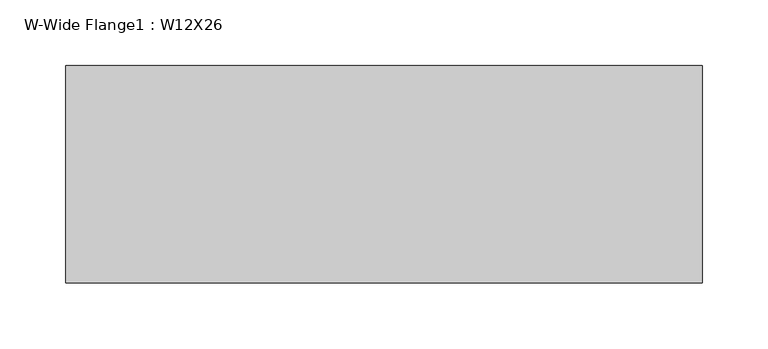
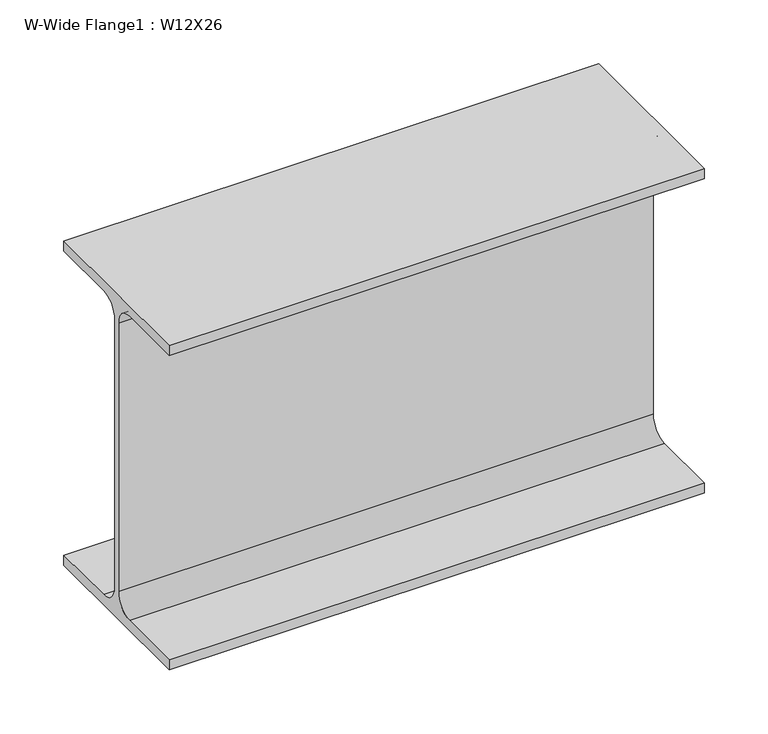
"""IFC4 building model written with IfcOpenShell, lengths in millimetres: beam geometry, W-Wide Flange1 : W12X26."""

import ifcopenshell
import ifcopenshell.guid

model = None  # the IFC model being written
_history = None  # IfcOwnerHistory: only IFC2X3 demands one
_inside = {}  # id of a spatial element -> (the spatial element, [elements in it])
_under = {}  # id of a project, library or spatial element -> (it, [spatial elements below it])
_declared = {}  # id of a project -> (the project, [libraries it declares])
_typed = {}  # id of a type object -> (the type object, [elements of that type])
_made_of = {}  # id of a material, layer set ... -> (it, [elements and type objects made of it])


def new_model(schema):
    """Start an empty IFC model of exactly this schema.

    Asked for "IFC4X3", IfcOpenShell would pick the latest addendum, in which some entities
    have other attributes; the version numbers below select the first issue.
    IFC2X3 requires an IfcOwnerHistory on every rooted entity: one is made here for all.
    """
    global model, _history
    if schema == "IFC4X3":
        model = ifcopenshell.file(schema_version=(4, 3, 0, 0))
    else:
        model = ifcopenshell.file(schema=schema)
    _inside.clear()
    _under.clear()
    _declared.clear()
    _typed.clear()
    _made_of.clear()
    _history = None
    if model.schema == "IFC2X3":
        org = make("IfcOrganization", Name="unknown")
        user = make(
            "IfcPersonAndOrganization",
            ThePerson=make("IfcPerson", FamilyName="unknown"),
            TheOrganization=org,
        )
        app = make(
            "IfcApplication",
            ApplicationDeveloper=org,
            Version="unknown",
            ApplicationFullName="unknown",
            ApplicationIdentifier="unknown",
        )
        _history = make(
            "IfcOwnerHistory",
            OwningUser=user,
            OwningApplication=app,
            ChangeAction="ADDED",
            CreationDate=0,
        )
    return model


def make(cls, **values):
    """One entity of the class cls with the attributes given. An attribute that is None is left unset."""
    return model.create_entity(
        cls, **{name: value for name, value in values.items() if value is not None}
    )


def rooted(cls, **values):
    """An entity with a GlobalId (a new one), such as an element, a storey or a relation."""
    return make(cls, GlobalId=ifcopenshell.guid.new(), OwnerHistory=_history, **values)


def si_unit(unit_type, name, prefix=None):
    """IfcSIUnit, for example si_unit("LENGTHUNIT", "METRE", prefix="MILLI")."""
    return make("IfcSIUnit", UnitType=unit_type, Prefix=prefix, Name=name)


def assignment(units):
    """IfcUnitAssignment: the units of a project."""
    return None if units is None else make("IfcUnitAssignment", Units=units)


def point(xyz):
    """IfcCartesianPoint."""
    return None if xyz is None else make("IfcCartesianPoint", Coordinates=xyz)


def direction(xyz):
    """IfcDirection."""
    return None if xyz is None else make("IfcDirection", DirectionRatios=xyz)


def frame(location, z_axis=None, x_axis=None):
    """IfcAxis2Placement3D, a coordinate frame: its origin and axes. An axis left out is left unset."""
    return make(
        "IfcAxis2Placement3D",
        Location=point(location),
        Axis=direction(z_axis),
        RefDirection=direction(x_axis),
    )


def frame_2d(location, x_axis=None):
    """IfcAxis2Placement2D, a coordinate frame in the plane: its origin and x axis."""
    return make(
        "IfcAxis2Placement2D", Location=point(location), RefDirection=direction(x_axis)
    )


def origin():
    """The frame at (0, 0, 0) with its axes left unset."""
    return frame((0.0, 0.0, 0.0))


def place(relative_to, where):
    """IfcLocalPlacement: puts the frame where relative to a parent placement (None: the world)."""
    return make(
        "IfcLocalPlacement", PlacementRelTo=relative_to, RelativePlacement=where
    )


def context(
    kind, dimensions, precision=None, world=None, true_north=None, identifier=None
):
    """IfcGeometricRepresentationContext, for example the 3D "Model" context."""
    return make(
        "IfcGeometricRepresentationContext",
        ContextIdentifier=identifier,
        ContextType=kind,
        CoordinateSpaceDimension=dimensions,
        Precision=precision,
        WorldCoordinateSystem=world,
        TrueNorth=true_north,
    )


def project(units=None, contexts=None):
    """IfcProject with its units and contexts."""
    return rooted(
        "IfcProject",
        Name="project",
        RepresentationContexts=contexts,
        UnitsInContext=assignment(units),
    )


def spatial(cls, under=None, at=None, **own):
    """A site, building, storey or space (cls), placed at a placement, below another one or the project."""
    s = rooted(cls, ObjectPlacement=at, **own)
    if under is not None:
        _under.setdefault(under.id(), (under, []))[1].append(s)
    return s


def polyline(points):
    """IfcPolyline through the points."""
    return make("IfcPolyline", Points=[point(p) for p in points])


def circle_curve(where, radius):
    """IfcCircle in the frame where."""
    return make("IfcCircle", Position=where, Radius=radius)


def trimmed(basis, trim1, trim2, sense, master):
    """IfcTrimmedCurve: the piece of a basis curve between two trims."""
    return make(
        "IfcTrimmedCurve",
        BasisCurve=basis,
        Trim1=trim1,
        Trim2=trim2,
        SenseAgreement=sense,
        MasterRepresentation=master,
    )


def segment(curve, same_sense, transition):
    """IfcCompositeCurveSegment."""
    return make(
        "IfcCompositeCurveSegment",
        Transition=transition,
        SameSense=same_sense,
        ParentCurve=curve,
    )


def composite_curve(segments, self_intersect=None):
    """IfcCompositeCurve: segments joined end to end."""
    return make("IfcCompositeCurve", Segments=segments, SelfIntersect=self_intersect)


def outline(outer, holes=None, kind="AREA"):
    """IfcArbitraryClosedProfileDef: a profile drawn as a closed curve; with holes, ...WithVoids."""
    if holes is None:
        return make("IfcArbitraryClosedProfileDef", ProfileType=kind, OuterCurve=outer)
    return make(
        "IfcArbitraryProfileDefWithVoids",
        ProfileType=kind,
        OuterCurve=outer,
        InnerCurves=holes,
    )


def extrude(swept, where, along, depth):
    """IfcExtrudedAreaSolid: the profile swept, set in the frame where, extruded along a direction by depth."""
    return make(
        "IfcExtrudedAreaSolid",
        SweptArea=swept,
        Position=where,
        ExtrudedDirection=direction(along),
        Depth=depth,
    )


def shape(context_of_items, identifier, shape_type, items):
    """IfcShapeRepresentation: the items that make up one representation, for example the "Body"."""
    return make(
        "IfcShapeRepresentation",
        ContextOfItems=context_of_items,
        RepresentationIdentifier=identifier,
        RepresentationType=shape_type,
        Items=items,
    )


def source(mapping_origin, context_of_items, identifier, shape_type, items):
    """IfcRepresentationMap: a shape defined once, which mapped items show again and again."""
    return make(
        "IfcRepresentationMap",
        MappingOrigin=mapping_origin,
        MappedRepresentation=shape(context_of_items, identifier, shape_type, items),
    )


def transform(
    local_origin,
    x_axis=None,
    y_axis=None,
    z_axis=None,
    scale=None,
    scale2=None,
    scale3=None,
    uniform=True,
):
    """IfcCartesianTransformationOperator3D, or its non-uniform kind. x_axis, y_axis, z_axis: its Axis1, 2, 3."""
    if uniform:
        return make(
            "IfcCartesianTransformationOperator3D",
            Axis1=direction(x_axis),
            Axis2=direction(y_axis),
            LocalOrigin=point(local_origin),
            Scale=scale,
            Axis3=direction(z_axis),
        )
    return make(
        "IfcCartesianTransformationOperator3DnonUniform",
        Axis1=direction(x_axis),
        Axis2=direction(y_axis),
        LocalOrigin=point(local_origin),
        Scale=scale,
        Axis3=direction(z_axis),
        Scale2=scale2,
        Scale3=scale3,
    )


def mapped(mapping_source, mapping_target):
    """IfcMappedItem: shows the shape of a source again, moved by a transform."""
    return make(
        "IfcMappedItem", MappingSource=mapping_source, MappingTarget=mapping_target
    )


def made_of(thing, what):
    """Note that an element or type object is made of a material, layer set ...; save() writes the relation."""
    if what is not None:
        _made_of.setdefault(what.id(), (what, []))[1].append(thing)
    return thing


def element(
    cls,
    number,
    at=None,
    inside=None,
    cuts=None,
    type_object=None,
    material=None,
    context=None,
    identifier="Body",
    shape_type=None,
    held_by="IfcProductDefinitionShape",
    body=None,
    shapes=None,
    **own,
):
    """One element of the class cls, such as IfcWall. Its Tag is "e" and its number.

    at: its placement. inside: the storey or other place that contains it. cuts: it is an
    opening in that element (IfcRelVoidsElement). A single representation is given by context,
    identifier, shape_type and body (its items); several are given by shapes. held_by: the class
    of the entity that holds the representations. save() writes the other relations.
    """
    e = rooted(cls, Tag="e%d" % number, ObjectPlacement=at, **own)
    if body is not None:
        shapes = [shape(context, identifier, shape_type, body)]
    if shapes is not None:
        e.Representation = make(held_by, Representations=shapes)
    if inside is not None:
        _inside.setdefault(inside.id(), (inside, []))[1].append(e)
    if cuts is not None:
        rooted(
            "IfcRelVoidsElement", RelatingBuildingElement=cuts, RelatedOpeningElement=e
        )
    if type_object is not None:
        _typed.setdefault(type_object.id(), (type_object, []))[1].append(e)
    return made_of(e, material)


def aggregate(whole, parts):
    """IfcRelAggregates: a whole, such as a stair, and the parts it consists of."""
    return rooted("IfcRelAggregates", RelatingObject=whole, RelatedObjects=parts)


def save(model, path):
    """Write the relations noted so far, then the file.

    IfcRelAggregates (storeys below a building ...), IfcRelContainedInSpatialStructure (elements
    in a storey), IfcRelDefinesByType, IfcRelAssociatesMaterial and IfcRelDeclares: one each for
    every whole, place, type object, material and project.
    """
    for whole, parts in _under.values():
        aggregate(whole, parts)
    for where, things in _inside.values():
        rooted(
            "IfcRelContainedInSpatialStructure",
            RelatedElements=things,
            RelatingStructure=where,
        )
    for kind, things in _typed.values():
        rooted("IfcRelDefinesByType", RelatedObjects=things, RelatingType=kind)
    for what, things in _made_of.values():
        rooted("IfcRelAssociatesMaterial", RelatedObjects=things, RelatingMaterial=what)
    for by, libraries in _declared.values():
        rooted("IfcRelDeclares", RelatingContext=by, RelatedDefinitions=libraries)
    model.write(path)


def w_wide_flange1_w12x26_d4e96f5b(model_context):
    return source(origin(), model_context, "Body", "SweptSolid", [
        extrude(outline(composite_curve([segment(polyline([(82.423, -145.288), (82.423, -154.94), (-82.423, -154.94), (-82.423, -145.288), (-20.2565, -145.288)]), True, "CONTINUOUS"), segment(trimmed(circle_curve(frame_2d((-20.2565, -127.9525)), 17.3355), [point((-20.2565, -145.288))], [point((-2.921, -127.9525))], True, "CARTESIAN"), True, "CONTINUOUS"), segment(polyline([(-2.921, -127.9525), (-2.921, 127.9525)]), True, "CONTINUOUS"), segment(trimmed(circle_curve(frame_2d((-20.2565, 127.9525)), 17.3355), [point((-2.921, 127.9525))], [point((-20.2565, 145.288))], True, "CARTESIAN"), True, "CONTINUOUS"), segment(polyline([(-20.2565, 145.288), (-82.423, 145.288), (-82.423, 154.94), (82.423, 154.94), (82.423, 145.288), (20.2565, 145.288)]), True, "CONTINUOUS"), segment(trimmed(circle_curve(frame_2d((20.2565, 127.9525)), 17.3355), [point((20.2565, 145.288))], [point((2.921, 127.9525))], True, "CARTESIAN"), True, "CONTINUOUS"), segment(polyline([(2.921, 127.9525), (2.921, -127.9525)]), True, "CONTINUOUS"), segment(trimmed(circle_curve(frame_2d((20.2565, -127.9525)), 17.3355), [point((2.921, -127.9525))], [point((20.2565, -145.288))], True, "CARTESIAN"), True, "CONTINUOUS"), segment(polyline([(20.2565, -145.288), (82.423, -145.288)]), True, "CONTINUOUS")], self_intersect=False)), frame((-229.2533826, 0.0, 0.0), z_axis=(1.0, 0.0, 0.0), x_axis=(0.0, 1.0, 0.0)), (0.0, 0.0, 1.0), 482.8463281),
    ])


if __name__ == "__main__":
    model = new_model("IFC4")
    model_context = context("Model", 3, world=origin())
    ifc_project = project(units=[si_unit("LENGTHUNIT", "METRE", prefix="MILLI")], contexts=[model_context])
    site = spatial("IfcSite", under=ifc_project)
    building = spatial("IfcBuilding", under=site)
    placement = place(None, origin())
    w_wide_flange1_w12x26_shape = w_wide_flange1_w12x26_d4e96f5b(model_context)
    element("IfcBeam", 1, ObjectType="W-Wide Flange1 : W12X26", at=placement, inside=building, context=model_context, shape_type="MappedRepresentation", body=[
        mapped(w_wide_flange1_w12x26_shape, transform((0.0, 0.0, 0.0), x_axis=(1.0, 0.0, 0.0), y_axis=(0.0, 1.0, 0.0), z_axis=(0.0, 0.0, 1.0))),
    ])
    save(model, "model.ifc")

# Revit data of these elements
# Type "W-Wide Flange1 : W12X26"
#   Assembly Code = "B10"
#   W = 26
#   Start Extension Calculation [instance default] = 10' - 0"
#   Start Extension [instance default] = -0' - 0 1/2"
#   End Extension Calculation [instance default] = 10' - 0"
#   End Extension [instance default] = -0' - 0 1/2"
#   Length [instance default] = 5' - 0"
#   bf = 0' - 6.49"
#   d = 1' - 0.2"
#   k = 0' - 1 1/16"
#   k2 = 0' - 0.6825"
#   tf = 0' - 0.38"
#   tw = 0' - 0.23"
#   A = 0.053125 SF
#   Structural Material [instance default] = Metal - Steel - ASTM A992
# Element 1 (IfcBeam, "W-Wide Flange1 : W12X26")
#   Materials on its faces: "Metal - Steel - ASTM A992"
# Materials
#   "Metal - Steel - ASTM A992": class "Metal", colour RGB 199 199 199, transparency 0
